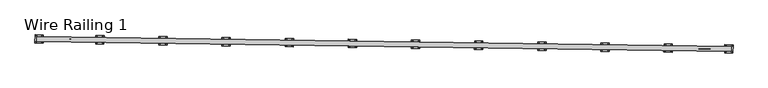
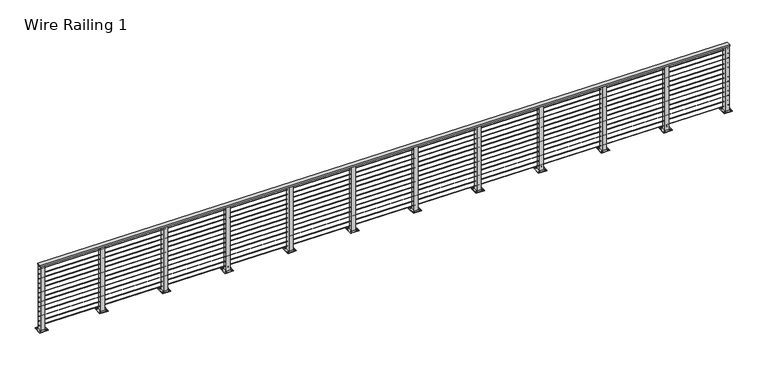
"""IFC4 building model written with IfcOpenShell, lengths in millimetres: railing geometry, Wire Railing 1."""

from ifc_helpers import new_model, si_unit, point, frame, frame_2d, origin, place, context, project, spatial, polyline, circle_curve, trimmed, segment, composite_curve, outline, extrude, source, transform, mapped, element, save


def wire_railing_1_a902e167(model_context):
    return source(origin(), model_context, "Body", "SweptSolid", [
        extrude(outline(polyline([(35445.2454193, 41277.4063498), (35446.3492316, 41353.5983546), (45957.1135693, 41201.326324), (45956.009757, 41125.1343191), (35445.2454193, 41277.4063498)])), frame((0.0, 0.0, 267138.15), z_axis=(0.0, 0.0, 1.0), x_axis=(1.0, 0.0, 0.0)), (0.0, 0.0, 1.0), 19.05),
        extrude(outline(composite_curve([segment(trimmed(circle_curve(frame_2d((0.0, 2.38125)), 2.38125), [point((2.3812499, 2.38125))], [point((-2.3812501, 2.38125))], False, "CARTESIAN"), True, "CONTINUOUS"), segment(trimmed(circle_curve(frame_2d((0.0, 2.38125)), 2.38125), [point((-2.3812501, 2.38125))], [point((2.3812499, 2.38125))], False, "CARTESIAN"), True, "CONTINUOUS")], self_intersect=False)), frame((45956.5616632, 41163.2303216, 267081.0), z_axis=(-0.9998950763646337, 0.014485726138629394, 0.0), x_axis=(0.014485726138629394, 0.9998950763646337, 0.0)), (0.0, 0.0, 1.0), 10511.8672811),
        extrude(outline(composite_curve([segment(trimmed(circle_curve(frame_2d((0.0, 2.38125)), 2.38125), [point((2.3812499, 2.38125))], [point((-2.3812501, 2.38125))], False, "CARTESIAN"), True, "CONTINUOUS"), segment(trimmed(circle_curve(frame_2d((0.0, 2.38125)), 2.38125), [point((-2.3812501, 2.38125))], [point((2.3812499, 2.38125))], False, "CARTESIAN"), True, "CONTINUOUS")], self_intersect=False)), frame((45956.5616632, 41163.2303216, 267004.8), z_axis=(-0.9998950763646337, 0.014485726138629394, 0.0), x_axis=(0.014485726138629394, 0.9998950763646337, 0.0)), (0.0, 0.0, 1.0), 10511.8672811),
        extrude(outline(composite_curve([segment(trimmed(circle_curve(frame_2d((0.0, 2.38125)), 2.38125), [point((2.3812499, 2.38125))], [point((-2.3812501, 2.38125))], False, "CARTESIAN"), True, "CONTINUOUS"), segment(trimmed(circle_curve(frame_2d((0.0, 2.38125)), 2.38125), [point((-2.3812501, 2.38125))], [point((2.3812499, 2.38125))], False, "CARTESIAN"), True, "CONTINUOUS")], self_intersect=False)), frame((45956.5616632, 41163.2303216, 266928.6), z_axis=(-0.9998950763646337, 0.014485726138629394, 0.0), x_axis=(0.014485726138629394, 0.9998950763646337, 0.0)), (0.0, 0.0, 1.0), 10511.8672811),
        extrude(outline(composite_curve([segment(trimmed(circle_curve(frame_2d((0.0, 2.38125)), 2.38125), [point((2.3812499, 2.38125))], [point((-2.3812501, 2.38125))], False, "CARTESIAN"), True, "CONTINUOUS"), segment(trimmed(circle_curve(frame_2d((0.0, 2.38125)), 2.38125), [point((-2.3812501, 2.38125))], [point((2.3812499, 2.38125))], False, "CARTESIAN"), True, "CONTINUOUS")], self_intersect=False)), frame((45956.5616632, 41163.2303216, 266852.4), z_axis=(-0.9998950763646337, 0.014485726138629394, 0.0), x_axis=(0.014485726138629394, 0.9998950763646337, 0.0)), (0.0, 0.0, 1.0), 10511.8672811),
        extrude(outline(composite_curve([segment(trimmed(circle_curve(frame_2d((0.0, 2.38125)), 2.38125), [point((2.3812499, 2.38125))], [point((-2.3812501, 2.38125))], False, "CARTESIAN"), True, "CONTINUOUS"), segment(trimmed(circle_curve(frame_2d((0.0, 2.38125)), 2.38125), [point((-2.3812501, 2.38125))], [point((2.3812499, 2.38125))], False, "CARTESIAN"), True, "CONTINUOUS")], self_intersect=False)), frame((45956.5616632, 41163.2303216, 266776.2), z_axis=(-0.9998950763646337, 0.014485726138629394, 0.0), x_axis=(0.014485726138629394, 0.9998950763646337, 0.0)), (0.0, 0.0, 1.0), 10511.8672811),
        extrude(outline(composite_curve([segment(trimmed(circle_curve(frame_2d((0.0, 2.38125)), 2.38125), [point((2.3812499, 2.38125))], [point((-2.3812501, 2.38125))], False, "CARTESIAN"), True, "CONTINUOUS"), segment(trimmed(circle_curve(frame_2d((0.0, 2.38125)), 2.38125), [point((-2.3812501, 2.38125))], [point((2.3812499, 2.38125))], False, "CARTESIAN"), True, "CONTINUOUS")], self_intersect=False)), frame((45956.5616632, 41163.2303216, 266700.0), z_axis=(-0.9998950763646337, 0.014485726138629394, 0.0), x_axis=(0.014485726138629394, 0.9998950763646337, 0.0)), (0.0, 0.0, 1.0), 10511.8672811),
        extrude(outline(composite_curve([segment(trimmed(circle_curve(frame_2d((0.0, 2.38125)), 2.38125), [point((2.3812499, 2.38125))], [point((-2.3812501, 2.38125))], False, "CARTESIAN"), True, "CONTINUOUS"), segment(trimmed(circle_curve(frame_2d((0.0, 2.38125)), 2.38125), [point((-2.3812501, 2.38125))], [point((2.3812499, 2.38125))], False, "CARTESIAN"), True, "CONTINUOUS")], self_intersect=False)), frame((45956.5616632, 41163.2303216, 266623.8), z_axis=(-0.9998950763646337, 0.014485726138629394, 0.0), x_axis=(0.014485726138629394, 0.9998950763646337, 0.0)), (0.0, 0.0, 1.0), 10511.8672811),
        extrude(outline(composite_curve([segment(trimmed(circle_curve(frame_2d((0.0, 2.38125)), 2.38125), [point((2.3812499, 2.38125))], [point((-2.3812501, 2.38125))], False, "CARTESIAN"), True, "CONTINUOUS"), segment(trimmed(circle_curve(frame_2d((0.0, 2.38125)), 2.38125), [point((-2.3812501, 2.38125))], [point((2.3812499, 2.38125))], False, "CARTESIAN"), True, "CONTINUOUS")], self_intersect=False)), frame((45956.5616632, 41163.2303216, 266547.6), z_axis=(-0.9998950763646337, 0.014485726138629394, 0.0), x_axis=(0.014485726138629394, 0.9998950763646337, 0.0)), (0.0, 0.0, 1.0), 10511.8672811),
        extrude(outline(composite_curve([segment(trimmed(circle_curve(frame_2d((0.0, 2.38125)), 2.38125), [point((2.3812499, 2.38125))], [point((-2.3812501, 2.38125))], False, "CARTESIAN"), True, "CONTINUOUS"), segment(trimmed(circle_curve(frame_2d((0.0, 2.38125)), 2.38125), [point((-2.3812501, 2.38125))], [point((2.3812499, 2.38125))], False, "CARTESIAN"), True, "CONTINUOUS")], self_intersect=False)), frame((45956.5616632, 41163.2303216, 266471.4), z_axis=(-0.9998950763646337, 0.014485726138629394, 0.0), x_axis=(0.014485726138629394, 0.9998950763646337, 0.0)), (0.0, 0.0, 1.0), 10511.8672811),
        extrude(outline(composite_curve([segment(trimmed(circle_curve(frame_2d((0.0, 2.38125)), 2.38125), [point((2.3812499, 2.38125))], [point((-2.3812501, 2.38125))], False, "CARTESIAN"), True, "CONTINUOUS"), segment(trimmed(circle_curve(frame_2d((0.0, 2.38125)), 2.38125), [point((-2.3812501, 2.38125))], [point((2.3812499, 2.38125))], False, "CARTESIAN"), True, "CONTINUOUS")], self_intersect=False)), frame((45956.5616632, 41163.2303216, 266395.2), z_axis=(-0.9998950763646337, 0.014485726138629394, 0.0), x_axis=(0.014485726138629394, 0.9998950763646337, 0.0)), (0.0, 0.0, 1.0), 10511.8672811),
        extrude(outline(composite_curve([segment(trimmed(circle_curve(frame_2d((0.0, 2.38125)), 2.38125), [point((2.3812499, 2.38125))], [point((-2.3812501, 2.38125))], False, "CARTESIAN"), True, "CONTINUOUS"), segment(trimmed(circle_curve(frame_2d((0.0, 2.38125)), 2.38125), [point((-2.3812501, 2.38125))], [point((2.3812499, 2.38125))], False, "CARTESIAN"), True, "CONTINUOUS")], self_intersect=False)), frame((45956.5616632, 41163.2303216, 266319.0), z_axis=(-0.9998950763646337, 0.014485726138629394, 0.0), x_axis=(0.014485726138629394, 0.9998950763646337, 0.0)), (0.0, 0.0, 1.0), 10511.8672811),
        extrude(outline(composite_curve([segment(trimmed(circle_curve(frame_2d((0.0, 2.38125)), 2.38125), [point((2.3812499, 2.38125))], [point((-2.3812501, 2.38125))], False, "CARTESIAN"), True, "CONTINUOUS"), segment(trimmed(circle_curve(frame_2d((0.0, 2.38125)), 2.38125), [point((-2.3812501, 2.38125))], [point((2.3812499, 2.38125))], False, "CARTESIAN"), True, "CONTINUOUS")], self_intersect=False)), frame((45956.5616632, 41163.2303216, 266242.8), z_axis=(-0.9998950763646337, 0.014485726138629394, 0.0), x_axis=(0.014485726138629394, 0.9998950763646337, 0.0)), (0.0, 0.0, 1.0), 10511.8672811),
        extrude(outline(composite_curve([segment(trimmed(circle_curve(frame_2d((0.0, 2.38125)), 2.38125), [point((2.3812499, 2.38125))], [point((-2.3812501, 2.38125))], False, "CARTESIAN"), True, "CONTINUOUS"), segment(trimmed(circle_curve(frame_2d((0.0, 2.38125)), 2.38125), [point((-2.3812501, 2.38125))], [point((2.3812499, 2.38125))], False, "CARTESIAN"), True, "CONTINUOUS")], self_intersect=False)), frame((45956.5616632, 41163.2303216, 266166.6), z_axis=(-0.9998950763646337, 0.014485726138629394, 0.0), x_axis=(0.014485726138629394, 0.9998950763646337, 0.0)), (0.0, 0.0, 1.0), 10511.8672811),
        extrude(outline(composite_curve([segment(trimmed(circle_curve(frame_2d((44955.9484058, 41133.2717878)), 6.35), [point((44955.8564214, 41126.9224541))], [point((44956.0403902, 41139.6211215))], False, "CARTESIAN"), True, "CONTINUOUS"), segment(trimmed(circle_curve(frame_2d((44955.9484058, 41133.2717878)), 6.35), [point((44956.0403902, 41139.6211215))], [point((44955.8564214, 41126.9224541))], False, "CARTESIAN"), True, "CONTINUOUS")], self_intersect=False)), frame((0.0, 0.0, 266090.4), z_axis=(0.0, 0.0, 1.0), x_axis=(1.0, 0.0, 0.0)), (0.0, 0.0, 1.0), 12.7),
        extrude(outline(composite_curve([segment(trimmed(circle_curve(frame_2d((44957.2361869, 41222.1624601)), 6.35), [point((44957.1442025, 41215.8131264))], [point((44957.3281712, 41228.5117938))], False, "CARTESIAN"), True, "CONTINUOUS"), segment(trimmed(circle_curve(frame_2d((44957.2361869, 41222.1624601)), 6.35), [point((44957.3281712, 41228.5117938))], [point((44957.1442025, 41215.8131264))], False, "CARTESIAN"), True, "CONTINUOUS")], self_intersect=False)), frame((0.0, 0.0, 266090.4), z_axis=(0.0, 0.0, 1.0), x_axis=(1.0, 0.0, 0.0)), (0.0, 0.0, 1.0), 12.7),
        extrude(outline(composite_curve([segment(trimmed(circle_curve(frame_2d((45044.8390781, 41131.9840068)), 6.35), [point((45044.7470937, 41125.634673))], [point((45044.9310624, 41138.3333405))], False, "CARTESIAN"), True, "CONTINUOUS"), segment(trimmed(circle_curve(frame_2d((45044.8390781, 41131.9840068)), 6.35), [point((45044.9310624, 41138.3333405))], [point((45044.7470937, 41125.634673))], False, "CARTESIAN"), True, "CONTINUOUS")], self_intersect=False)), frame((0.0, 0.0, 266090.4), z_axis=(0.0, 0.0, 1.0), x_axis=(1.0, 0.0, 0.0)), (0.0, 0.0, 1.0), 12.7),
        extrude(outline(composite_curve([segment(trimmed(circle_curve(frame_2d((45046.1268591, 41220.874679)), 6.35), [point((45046.0348748, 41214.5253453))], [point((45046.2188435, 41227.2240128))], False, "CARTESIAN"), True, "CONTINUOUS"), segment(trimmed(circle_curve(frame_2d((45046.1268591, 41220.874679)), 6.35), [point((45046.2188435, 41227.2240128))], [point((45046.0348748, 41214.5253453))], False, "CARTESIAN"), True, "CONTINUOUS")], self_intersect=False)), frame((0.0, 0.0, 266090.4), z_axis=(0.0, 0.0, 1.0), x_axis=(1.0, 0.0, 0.0)), (0.0, 0.0, 1.0), 12.7),
        extrude(outline(polyline([(44938.4641387, 41241.4864144), (45065.4508134, 41239.6467272), (45063.6111262, 41112.6600525), (44936.6244515, 41114.4997397), (44938.4641387, 41241.4864144)])), frame((0.0, 0.0, 266090.4), z_axis=(0.0, 0.0, 1.0), x_axis=(1.0, 0.0, 0.0)), (0.0, 0.0, 1.0), 6.35),
        extrude(outline(polyline([(44971.3152229, 41207.6694944), (45031.6338934, 41206.795643), (45030.760042, 41146.4769725), (44970.4413715, 41147.3508239), (44971.3152229, 41207.6694944)]), holes=[polyline([(44977.5725723, 41201.2281763), (44976.8826896, 41153.6081733), (45024.5026926, 41152.9182906), (45025.1925753, 41200.5382936), (44977.5725723, 41201.2281763)])]), frame((0.0, 0.0, 266090.4), z_axis=(0.0, 0.0, 1.0), x_axis=(1.0, 0.0, 0.0)), (0.0, 0.0, 1.0), 1047.75),
        extrude(outline(composite_curve([segment(trimmed(circle_curve(frame_2d((44000.4243751, 41147.1146997)), 6.35), [point((44000.3323907, 41140.765366))], [point((44000.5163595, 41153.4640334))], False, "CARTESIAN"), True, "CONTINUOUS"), segment(trimmed(circle_curve(frame_2d((44000.4243751, 41147.1146997)), 6.35), [point((44000.5163595, 41153.4640334))], [point((44000.3323907, 41140.765366))], False, "CARTESIAN"), True, "CONTINUOUS")], self_intersect=False)), frame((0.0, 0.0, 266090.4), z_axis=(0.0, 0.0, 1.0), x_axis=(1.0, 0.0, 0.0)), (0.0, 0.0, 1.0), 12.7),
        extrude(outline(composite_curve([segment(trimmed(circle_curve(frame_2d((44001.7121561, 41236.005372)), 6.35), [point((44001.6201718, 41229.6560382))], [point((44001.8041405, 41242.3547057))], False, "CARTESIAN"), True, "CONTINUOUS"), segment(trimmed(circle_curve(frame_2d((44001.7121561, 41236.005372)), 6.35), [point((44001.8041405, 41242.3547057))], [point((44001.6201718, 41229.6560382))], False, "CARTESIAN"), True, "CONTINUOUS")], self_intersect=False)), frame((0.0, 0.0, 266090.4), z_axis=(0.0, 0.0, 1.0), x_axis=(1.0, 0.0, 0.0)), (0.0, 0.0, 1.0), 12.7),
        extrude(outline(composite_curve([segment(trimmed(circle_curve(frame_2d((44089.3150474, 41145.8269186)), 6.35), [point((44089.223063, 41139.4775849))], [point((44089.4070317, 41152.1762524))], False, "CARTESIAN"), True, "CONTINUOUS"), segment(trimmed(circle_curve(frame_2d((44089.3150474, 41145.8269186)), 6.35), [point((44089.4070317, 41152.1762524))], [point((44089.223063, 41139.4775849))], False, "CARTESIAN"), True, "CONTINUOUS")], self_intersect=False)), frame((0.0, 0.0, 266090.4), z_axis=(0.0, 0.0, 1.0), x_axis=(1.0, 0.0, 0.0)), (0.0, 0.0, 1.0), 12.7),
        extrude(outline(composite_curve([segment(trimmed(circle_curve(frame_2d((44090.6028284, 41234.7175909)), 6.35), [point((44090.5108441, 41228.3682572))], [point((44090.6948128, 41241.0669247))], False, "CARTESIAN"), True, "CONTINUOUS"), segment(trimmed(circle_curve(frame_2d((44090.6028284, 41234.7175909)), 6.35), [point((44090.6948128, 41241.0669247))], [point((44090.5108441, 41228.3682572))], False, "CARTESIAN"), True, "CONTINUOUS")], self_intersect=False)), frame((0.0, 0.0, 266090.4), z_axis=(0.0, 0.0, 1.0), x_axis=(1.0, 0.0, 0.0)), (0.0, 0.0, 1.0), 12.7),
        extrude(outline(polyline([(43982.940108, 41255.3293263), (44109.9267827, 41253.489639), (44108.0870955, 41126.5029643), (43981.1004208, 41128.3426516), (43982.940108, 41255.3293263)])), frame((0.0, 0.0, 266090.4), z_axis=(0.0, 0.0, 1.0), x_axis=(1.0, 0.0, 0.0)), (0.0, 0.0, 1.0), 6.35),
        extrude(outline(polyline([(44015.7911922, 41221.5124063), (44076.1098627, 41220.6385548), (44075.2360113, 41160.3198844), (44014.9173408, 41161.1937358), (44015.7911922, 41221.5124063)]), holes=[polyline([(44022.0485416, 41215.0710882), (44021.3586589, 41167.4510852), (44068.9786619, 41166.7612024), (44069.6685446, 41214.3812055), (44022.0485416, 41215.0710882)])]), frame((0.0, 0.0, 266090.4), z_axis=(0.0, 0.0, 1.0), x_axis=(1.0, 0.0, 0.0)), (0.0, 0.0, 1.0), 1047.75),
        extrude(outline(composite_curve([segment(trimmed(circle_curve(frame_2d((43044.9003444, 41160.9576116)), 6.35), [point((43044.80836, 41154.6082778))], [point((43044.9923287, 41167.3069453))], False, "CARTESIAN"), True, "CONTINUOUS"), segment(trimmed(circle_curve(frame_2d((43044.9003444, 41160.9576116)), 6.35), [point((43044.9923287, 41167.3069453))], [point((43044.80836, 41154.6082778))], False, "CARTESIAN"), True, "CONTINUOUS")], self_intersect=False)), frame((0.0, 0.0, 266090.4), z_axis=(0.0, 0.0, 1.0), x_axis=(1.0, 0.0, 0.0)), (0.0, 0.0, 1.0), 12.7),
        extrude(outline(composite_curve([segment(trimmed(circle_curve(frame_2d((43046.1881254, 41249.8482839)), 6.35), [point((43046.0961411, 41243.4989501))], [point((43046.2801098, 41256.1976176))], False, "CARTESIAN"), True, "CONTINUOUS"), segment(trimmed(circle_curve(frame_2d((43046.1881254, 41249.8482839)), 6.35), [point((43046.2801098, 41256.1976176))], [point((43046.0961411, 41243.4989501))], False, "CARTESIAN"), True, "CONTINUOUS")], self_intersect=False)), frame((0.0, 0.0, 266090.4), z_axis=(0.0, 0.0, 1.0), x_axis=(1.0, 0.0, 0.0)), (0.0, 0.0, 1.0), 12.7),
        extrude(outline(composite_curve([segment(trimmed(circle_curve(frame_2d((43133.7910167, 41159.6698305)), 6.35), [point((43133.6990323, 41153.3204968))], [point((43133.883001, 41166.0191642))], False, "CARTESIAN"), True, "CONTINUOUS"), segment(trimmed(circle_curve(frame_2d((43133.7910167, 41159.6698305)), 6.35), [point((43133.883001, 41166.0191642))], [point((43133.6990323, 41153.3204968))], False, "CARTESIAN"), True, "CONTINUOUS")], self_intersect=False)), frame((0.0, 0.0, 266090.4), z_axis=(0.0, 0.0, 1.0), x_axis=(1.0, 0.0, 0.0)), (0.0, 0.0, 1.0), 12.7),
        extrude(outline(composite_curve([segment(trimmed(circle_curve(frame_2d((43135.0787977, 41248.5605028)), 6.35), [point((43134.9868134, 41242.2111691))], [point((43135.1707821, 41254.9098365))], False, "CARTESIAN"), True, "CONTINUOUS"), segment(trimmed(circle_curve(frame_2d((43135.0787977, 41248.5605028)), 6.35), [point((43135.1707821, 41254.9098365))], [point((43134.9868134, 41242.2111691))], False, "CARTESIAN"), True, "CONTINUOUS")], self_intersect=False)), frame((0.0, 0.0, 266090.4), z_axis=(0.0, 0.0, 1.0), x_axis=(1.0, 0.0, 0.0)), (0.0, 0.0, 1.0), 12.7),
        extrude(outline(polyline([(43027.4160773, 41269.1722381), (43154.402752, 41267.3325509), (43152.5630648, 41140.3458762), (43025.5763901, 41142.1855634), (43027.4160773, 41269.1722381)])), frame((0.0, 0.0, 266090.4), z_axis=(0.0, 0.0, 1.0), x_axis=(1.0, 0.0, 0.0)), (0.0, 0.0, 1.0), 6.35),
        extrude(outline(polyline([(43060.2671615, 41235.3553181), (43120.585832, 41234.4814667), (43119.7119806, 41174.1627962), (43059.3933101, 41175.0366477), (43060.2671615, 41235.3553181)]), holes=[polyline([(43066.5245109, 41228.914), (43065.8346282, 41181.293997), (43113.4546312, 41180.6041143), (43114.1445139, 41228.2241173), (43066.5245109, 41228.914)])]), frame((0.0, 0.0, 266090.4), z_axis=(0.0, 0.0, 1.0), x_axis=(1.0, 0.0, 0.0)), (0.0, 0.0, 1.0), 1047.75),
        extrude(outline(composite_curve([segment(trimmed(circle_curve(frame_2d((42089.3763137, 41174.8005234)), 6.35), [point((42089.2843293, 41168.4511897))], [point((42089.468298, 41181.1498572))], False, "CARTESIAN"), True, "CONTINUOUS"), segment(trimmed(circle_curve(frame_2d((42089.3763137, 41174.8005234)), 6.35), [point((42089.468298, 41181.1498572))], [point((42089.2843293, 41168.4511897))], False, "CARTESIAN"), True, "CONTINUOUS")], self_intersect=False)), frame((0.0, 0.0, 266090.4), z_axis=(0.0, 0.0, 1.0), x_axis=(1.0, 0.0, 0.0)), (0.0, 0.0, 1.0), 12.7),
        extrude(outline(composite_curve([segment(trimmed(circle_curve(frame_2d((42090.6640947, 41263.6911957)), 6.35), [point((42090.5721104, 41257.341862))], [point((42090.7560791, 41270.0405295))], False, "CARTESIAN"), True, "CONTINUOUS"), segment(trimmed(circle_curve(frame_2d((42090.6640947, 41263.6911957)), 6.35), [point((42090.7560791, 41270.0405295))], [point((42090.5721104, 41257.341862))], False, "CARTESIAN"), True, "CONTINUOUS")], self_intersect=False)), frame((0.0, 0.0, 266090.4), z_axis=(0.0, 0.0, 1.0), x_axis=(1.0, 0.0, 0.0)), (0.0, 0.0, 1.0), 12.7),
        extrude(outline(composite_curve([segment(trimmed(circle_curve(frame_2d((42178.266986, 41173.5127424)), 6.35), [point((42178.1750016, 41167.1634087))], [point((42178.3589703, 41179.8620761))], False, "CARTESIAN"), True, "CONTINUOUS"), segment(trimmed(circle_curve(frame_2d((42178.266986, 41173.5127424)), 6.35), [point((42178.3589703, 41179.8620761))], [point((42178.1750016, 41167.1634087))], False, "CARTESIAN"), True, "CONTINUOUS")], self_intersect=False)), frame((0.0, 0.0, 266090.4), z_axis=(0.0, 0.0, 1.0), x_axis=(1.0, 0.0, 0.0)), (0.0, 0.0, 1.0), 12.7),
        extrude(outline(composite_curve([segment(trimmed(circle_curve(frame_2d((42179.554767, 41262.4034147)), 6.35), [point((42179.4627827, 41256.0540809))], [point((42179.6467514, 41268.7527484))], False, "CARTESIAN"), True, "CONTINUOUS"), segment(trimmed(circle_curve(frame_2d((42179.554767, 41262.4034147)), 6.35), [point((42179.6467514, 41268.7527484))], [point((42179.4627827, 41256.0540809))], False, "CARTESIAN"), True, "CONTINUOUS")], self_intersect=False)), frame((0.0, 0.0, 266090.4), z_axis=(0.0, 0.0, 1.0), x_axis=(1.0, 0.0, 0.0)), (0.0, 0.0, 1.0), 12.7),
        extrude(outline(polyline([(42071.8920466, 41283.01515), (42198.8787213, 41281.1754628), (42197.0390341, 41154.1887881), (42070.0523594, 41156.0284753), (42071.8920466, 41283.01515)])), frame((0.0, 0.0, 266090.4), z_axis=(0.0, 0.0, 1.0), x_axis=(1.0, 0.0, 0.0)), (0.0, 0.0, 1.0), 6.35),
        extrude(outline(polyline([(42104.7431308, 41249.19823), (42165.0618013, 41248.3243786), (42164.1879499, 41188.0057081), (42103.8692794, 41188.8795595), (42104.7431308, 41249.19823)]), holes=[polyline([(42111.0004802, 41242.7569119), (42110.3105975, 41195.1369089), (42157.9306005, 41194.4470262), (42158.6204832, 41242.0670292), (42111.0004802, 41242.7569119)])]), frame((0.0, 0.0, 266090.4), z_axis=(0.0, 0.0, 1.0), x_axis=(1.0, 0.0, 0.0)), (0.0, 0.0, 1.0), 1047.75),
        extrude(outline(composite_curve([segment(trimmed(circle_curve(frame_2d((41133.852283, 41188.6434353)), 6.35), [point((41133.7602986, 41182.2941016))], [point((41133.9442673, 41194.9927691))], False, "CARTESIAN"), True, "CONTINUOUS"), segment(trimmed(circle_curve(frame_2d((41133.852283, 41188.6434353)), 6.35), [point((41133.9442673, 41194.9927691))], [point((41133.7602986, 41182.2941016))], False, "CARTESIAN"), True, "CONTINUOUS")], self_intersect=False)), frame((0.0, 0.0, 266090.4), z_axis=(0.0, 0.0, 1.0), x_axis=(1.0, 0.0, 0.0)), (0.0, 0.0, 1.0), 12.7),
        extrude(outline(composite_curve([segment(trimmed(circle_curve(frame_2d((41135.140064, 41277.5341076)), 6.35), [point((41135.0480797, 41271.1847739))], [point((41135.2320484, 41283.8834413))], False, "CARTESIAN"), True, "CONTINUOUS"), segment(trimmed(circle_curve(frame_2d((41135.140064, 41277.5341076)), 6.35), [point((41135.2320484, 41283.8834413))], [point((41135.0480797, 41271.1847739))], False, "CARTESIAN"), True, "CONTINUOUS")], self_intersect=False)), frame((0.0, 0.0, 266090.4), z_axis=(0.0, 0.0, 1.0), x_axis=(1.0, 0.0, 0.0)), (0.0, 0.0, 1.0), 12.7),
        extrude(outline(composite_curve([segment(trimmed(circle_curve(frame_2d((41222.7429553, 41187.3556543)), 6.35), [point((41222.6509709, 41181.0063205))], [point((41222.8349396, 41193.704988))], False, "CARTESIAN"), True, "CONTINUOUS"), segment(trimmed(circle_curve(frame_2d((41222.7429553, 41187.3556543)), 6.35), [point((41222.8349396, 41193.704988))], [point((41222.6509709, 41181.0063205))], False, "CARTESIAN"), True, "CONTINUOUS")], self_intersect=False)), frame((0.0, 0.0, 266090.4), z_axis=(0.0, 0.0, 1.0), x_axis=(1.0, 0.0, 0.0)), (0.0, 0.0, 1.0), 12.7),
        extrude(outline(composite_curve([segment(trimmed(circle_curve(frame_2d((41224.0307363, 41276.2463266)), 6.35), [point((41223.938752, 41269.8969928))], [point((41224.1227207, 41282.5956603))], False, "CARTESIAN"), True, "CONTINUOUS"), segment(trimmed(circle_curve(frame_2d((41224.0307363, 41276.2463266)), 6.35), [point((41224.1227207, 41282.5956603))], [point((41223.938752, 41269.8969928))], False, "CARTESIAN"), True, "CONTINUOUS")], self_intersect=False)), frame((0.0, 0.0, 266090.4), z_axis=(0.0, 0.0, 1.0), x_axis=(1.0, 0.0, 0.0)), (0.0, 0.0, 1.0), 12.7),
        extrude(outline(polyline([(41116.3680159, 41296.8580619), (41243.3546906, 41295.0183747), (41241.5150034, 41168.0317), (41114.5283287, 41169.8713872), (41116.3680159, 41296.8580619)])), frame((0.0, 0.0, 266090.4), z_axis=(0.0, 0.0, 1.0), x_axis=(1.0, 0.0, 0.0)), (0.0, 0.0, 1.0), 6.35),
        extrude(outline(polyline([(41149.2191001, 41263.0411419), (41209.5377706, 41262.1672905), (41208.6639192, 41201.84862), (41148.3452487, 41202.7224714), (41149.2191001, 41263.0411419)]), holes=[polyline([(41155.4764495, 41256.5998238), (41154.7865668, 41208.9798208), (41202.4065698, 41208.2899381), (41203.0964525, 41255.9099411), (41155.4764495, 41256.5998238)])]), frame((0.0, 0.0, 266090.4), z_axis=(0.0, 0.0, 1.0), x_axis=(1.0, 0.0, 0.0)), (0.0, 0.0, 1.0), 1047.75),
        extrude(outline(composite_curve([segment(trimmed(circle_curve(frame_2d((40178.3282523, 41202.4863472)), 6.35), [point((40178.2362679, 41196.1370135))], [point((40178.4202366, 41208.8356809))], False, "CARTESIAN"), True, "CONTINUOUS"), segment(trimmed(circle_curve(frame_2d((40178.3282523, 41202.4863472)), 6.35), [point((40178.4202366, 41208.8356809))], [point((40178.2362679, 41196.1370135))], False, "CARTESIAN"), True, "CONTINUOUS")], self_intersect=False)), frame((0.0, 0.0, 266090.4), z_axis=(0.0, 0.0, 1.0), x_axis=(1.0, 0.0, 0.0)), (0.0, 0.0, 1.0), 12.7),
        extrude(outline(composite_curve([segment(trimmed(circle_curve(frame_2d((40179.6160333, 41291.3770195)), 6.35), [point((40179.524049, 41285.0276857))], [point((40179.7080177, 41297.7263532))], False, "CARTESIAN"), True, "CONTINUOUS"), segment(trimmed(circle_curve(frame_2d((40179.6160333, 41291.3770195)), 6.35), [point((40179.7080177, 41297.7263532))], [point((40179.524049, 41285.0276857))], False, "CARTESIAN"), True, "CONTINUOUS")], self_intersect=False)), frame((0.0, 0.0, 266090.4), z_axis=(0.0, 0.0, 1.0), x_axis=(1.0, 0.0, 0.0)), (0.0, 0.0, 1.0), 12.7),
        extrude(outline(composite_curve([segment(trimmed(circle_curve(frame_2d((40267.2189246, 41201.1985661)), 6.35), [point((40267.1269402, 41194.8492324))], [point((40267.3109089, 41207.5478999))], False, "CARTESIAN"), True, "CONTINUOUS"), segment(trimmed(circle_curve(frame_2d((40267.2189246, 41201.1985661)), 6.35), [point((40267.3109089, 41207.5478999))], [point((40267.1269402, 41194.8492324))], False, "CARTESIAN"), True, "CONTINUOUS")], self_intersect=False)), frame((0.0, 0.0, 266090.4), z_axis=(0.0, 0.0, 1.0), x_axis=(1.0, 0.0, 0.0)), (0.0, 0.0, 1.0), 12.7),
        extrude(outline(composite_curve([segment(trimmed(circle_curve(frame_2d((40268.5067056, 41290.0892384)), 6.35), [point((40268.4147213, 41283.7399047))], [point((40268.59869, 41296.4385722))], False, "CARTESIAN"), True, "CONTINUOUS"), segment(trimmed(circle_curve(frame_2d((40268.5067056, 41290.0892384)), 6.35), [point((40268.59869, 41296.4385722))], [point((40268.4147213, 41283.7399047))], False, "CARTESIAN"), True, "CONTINUOUS")], self_intersect=False)), frame((0.0, 0.0, 266090.4), z_axis=(0.0, 0.0, 1.0), x_axis=(1.0, 0.0, 0.0)), (0.0, 0.0, 1.0), 12.7),
        extrude(outline(polyline([(40160.8439852, 41310.7009738), (40287.8306599, 41308.8612866), (40285.9909727, 41181.8746119), (40159.004298, 41183.7142991), (40160.8439852, 41310.7009738)])), frame((0.0, 0.0, 266090.4), z_axis=(0.0, 0.0, 1.0), x_axis=(1.0, 0.0, 0.0)), (0.0, 0.0, 1.0), 6.35),
        extrude(outline(polyline([(40193.6950694, 41276.8840538), (40254.0137399, 41276.0102023), (40253.1398885, 41215.6915319), (40192.821218, 41216.5653833), (40193.6950694, 41276.8840538)]), holes=[polyline([(40199.9524188, 41270.4427357), (40199.2625361, 41222.8227327), (40246.8825391, 41222.13285), (40247.5724218, 41269.752853), (40199.9524188, 41270.4427357)])]), frame((0.0, 0.0, 266090.4), z_axis=(0.0, 0.0, 1.0), x_axis=(1.0, 0.0, 0.0)), (0.0, 0.0, 1.0), 1047.75),
        extrude(outline(composite_curve([segment(trimmed(circle_curve(frame_2d((39222.8042216, 41216.3292591)), 6.35), [point((39222.7122372, 41209.9799253))], [point((39222.8962059, 41222.6785928))], False, "CARTESIAN"), True, "CONTINUOUS"), segment(trimmed(circle_curve(frame_2d((39222.8042216, 41216.3292591)), 6.35), [point((39222.8962059, 41222.6785928))], [point((39222.7122372, 41209.9799253))], False, "CARTESIAN"), True, "CONTINUOUS")], self_intersect=False)), frame((0.0, 0.0, 266090.4), z_axis=(0.0, 0.0, 1.0), x_axis=(1.0, 0.0, 0.0)), (0.0, 0.0, 1.0), 12.7),
        extrude(outline(composite_curve([segment(trimmed(circle_curve(frame_2d((39224.0920026, 41305.2199314)), 6.35), [point((39224.0000183, 41298.8705976))], [point((39224.183987, 41311.5692651))], False, "CARTESIAN"), True, "CONTINUOUS"), segment(trimmed(circle_curve(frame_2d((39224.0920026, 41305.2199314)), 6.35), [point((39224.183987, 41311.5692651))], [point((39224.0000183, 41298.8705976))], False, "CARTESIAN"), True, "CONTINUOUS")], self_intersect=False)), frame((0.0, 0.0, 266090.4), z_axis=(0.0, 0.0, 1.0), x_axis=(1.0, 0.0, 0.0)), (0.0, 0.0, 1.0), 12.7),
        extrude(outline(composite_curve([segment(trimmed(circle_curve(frame_2d((39311.6948939, 41215.041478)), 6.35), [point((39311.6029095, 41208.6921443))], [point((39311.7868782, 41221.3908118))], False, "CARTESIAN"), True, "CONTINUOUS"), segment(trimmed(circle_curve(frame_2d((39311.6948939, 41215.041478)), 6.35), [point((39311.7868782, 41221.3908118))], [point((39311.6029095, 41208.6921443))], False, "CARTESIAN"), True, "CONTINUOUS")], self_intersect=False)), frame((0.0, 0.0, 266090.4), z_axis=(0.0, 0.0, 1.0), x_axis=(1.0, 0.0, 0.0)), (0.0, 0.0, 1.0), 12.7),
        extrude(outline(composite_curve([segment(trimmed(circle_curve(frame_2d((39312.9826749, 41303.9321503)), 6.35), [point((39312.8906905, 41297.5828166))], [point((39313.0746593, 41310.281484))], False, "CARTESIAN"), True, "CONTINUOUS"), segment(trimmed(circle_curve(frame_2d((39312.9826749, 41303.9321503)), 6.35), [point((39313.0746593, 41310.281484))], [point((39312.8906905, 41297.5828166))], False, "CARTESIAN"), True, "CONTINUOUS")], self_intersect=False)), frame((0.0, 0.0, 266090.4), z_axis=(0.0, 0.0, 1.0), x_axis=(1.0, 0.0, 0.0)), (0.0, 0.0, 1.0), 12.7),
        extrude(outline(polyline([(39205.3199545, 41324.5438856), (39332.3066292, 41322.7041984), (39330.466942, 41195.7175237), (39203.4802673, 41197.5572109), (39205.3199545, 41324.5438856)])), frame((0.0, 0.0, 266090.4), z_axis=(0.0, 0.0, 1.0), x_axis=(1.0, 0.0, 0.0)), (0.0, 0.0, 1.0), 6.35),
        extrude(outline(polyline([(39238.1710387, 41290.7269656), (39298.4897092, 41289.8531142), (39297.6158578, 41229.5344437), (39237.2971873, 41230.4082952), (39238.1710387, 41290.7269656)]), holes=[polyline([(39244.4283881, 41284.2856475), (39243.7385054, 41236.6656445), (39291.3585084, 41235.9757618), (39292.0483911, 41283.5957648), (39244.4283881, 41284.2856475)])]), frame((0.0, 0.0, 266090.4), z_axis=(0.0, 0.0, 1.0), x_axis=(1.0, 0.0, 0.0)), (0.0, 0.0, 1.0), 1047.75),
        extrude(outline(composite_curve([segment(trimmed(circle_curve(frame_2d((38267.2801909, 41230.1721709)), 6.35), [point((38267.1882065, 41223.8228372))], [point((38267.3721752, 41236.5215047))], False, "CARTESIAN"), True, "CONTINUOUS"), segment(trimmed(circle_curve(frame_2d((38267.2801909, 41230.1721709)), 6.35), [point((38267.3721752, 41236.5215047))], [point((38267.1882065, 41223.8228372))], False, "CARTESIAN"), True, "CONTINUOUS")], self_intersect=False)), frame((0.0, 0.0, 266090.4), z_axis=(0.0, 0.0, 1.0), x_axis=(1.0, 0.0, 0.0)), (0.0, 0.0, 1.0), 12.7),
        extrude(outline(composite_curve([segment(trimmed(circle_curve(frame_2d((38268.5679719, 41319.0628432)), 6.35), [point((38268.4759876, 41312.7135095))], [point((38268.6599563, 41325.412177))], False, "CARTESIAN"), True, "CONTINUOUS"), segment(trimmed(circle_curve(frame_2d((38268.5679719, 41319.0628432)), 6.35), [point((38268.6599563, 41325.412177))], [point((38268.4759876, 41312.7135095))], False, "CARTESIAN"), True, "CONTINUOUS")], self_intersect=False)), frame((0.0, 0.0, 266090.4), z_axis=(0.0, 0.0, 1.0), x_axis=(1.0, 0.0, 0.0)), (0.0, 0.0, 1.0), 12.7),
        extrude(outline(composite_curve([segment(trimmed(circle_curve(frame_2d((38356.1708632, 41228.8843899)), 6.35), [point((38356.0788788, 41222.5350562))], [point((38356.2628475, 41235.2337236))], False, "CARTESIAN"), True, "CONTINUOUS"), segment(trimmed(circle_curve(frame_2d((38356.1708632, 41228.8843899)), 6.35), [point((38356.2628475, 41235.2337236))], [point((38356.0788788, 41222.5350562))], False, "CARTESIAN"), True, "CONTINUOUS")], self_intersect=False)), frame((0.0, 0.0, 266090.4), z_axis=(0.0, 0.0, 1.0), x_axis=(1.0, 0.0, 0.0)), (0.0, 0.0, 1.0), 12.7),
        extrude(outline(composite_curve([segment(trimmed(circle_curve(frame_2d((38357.4586442, 41317.7750622)), 6.35), [point((38357.3666598, 41311.4257284))], [point((38357.5506286, 41324.1243959))], False, "CARTESIAN"), True, "CONTINUOUS"), segment(trimmed(circle_curve(frame_2d((38357.4586442, 41317.7750622)), 6.35), [point((38357.5506286, 41324.1243959))], [point((38357.3666598, 41311.4257284))], False, "CARTESIAN"), True, "CONTINUOUS")], self_intersect=False)), frame((0.0, 0.0, 266090.4), z_axis=(0.0, 0.0, 1.0), x_axis=(1.0, 0.0, 0.0)), (0.0, 0.0, 1.0), 12.7),
        extrude(outline(polyline([(38249.7959238, 41338.3867975), (38376.7825985, 41336.5471103), (38374.9429113, 41209.5604356), (38247.9562366, 41211.4001228), (38249.7959238, 41338.3867975)])), frame((0.0, 0.0, 266090.4), z_axis=(0.0, 0.0, 1.0), x_axis=(1.0, 0.0, 0.0)), (0.0, 0.0, 1.0), 6.35),
        extrude(outline(polyline([(38282.647008, 41304.5698775), (38342.9656785, 41303.6960261), (38342.0918271, 41243.3773556), (38281.7731566, 41244.251207), (38282.647008, 41304.5698775)]), holes=[polyline([(38288.9043574, 41298.1285594), (38288.2144747, 41250.5085564), (38335.8344777, 41249.8186737), (38336.5243604, 41297.4386767), (38288.9043574, 41298.1285594)])]), frame((0.0, 0.0, 266090.4), z_axis=(0.0, 0.0, 1.0), x_axis=(1.0, 0.0, 0.0)), (0.0, 0.0, 1.0), 1047.75),
        extrude(outline(composite_curve([segment(trimmed(circle_curve(frame_2d((37311.7561602, 41244.0150828)), 6.35), [point((37311.6641758, 41237.6657491))], [point((37311.8481445, 41250.3644166))], False, "CARTESIAN"), True, "CONTINUOUS"), segment(trimmed(circle_curve(frame_2d((37311.7561602, 41244.0150828)), 6.35), [point((37311.8481445, 41250.3644166))], [point((37311.6641758, 41237.6657491))], False, "CARTESIAN"), True, "CONTINUOUS")], self_intersect=False)), frame((0.0, 0.0, 266090.4), z_axis=(0.0, 0.0, 1.0), x_axis=(1.0, 0.0, 0.0)), (0.0, 0.0, 1.0), 12.7),
        extrude(outline(composite_curve([segment(trimmed(circle_curve(frame_2d((37313.0439412, 41332.9057551)), 6.35), [point((37312.9519569, 41326.5564214))], [point((37313.1359256, 41339.2550888))], False, "CARTESIAN"), True, "CONTINUOUS"), segment(trimmed(circle_curve(frame_2d((37313.0439412, 41332.9057551)), 6.35), [point((37313.1359256, 41339.2550888))], [point((37312.9519569, 41326.5564214))], False, "CARTESIAN"), True, "CONTINUOUS")], self_intersect=False)), frame((0.0, 0.0, 266090.4), z_axis=(0.0, 0.0, 1.0), x_axis=(1.0, 0.0, 0.0)), (0.0, 0.0, 1.0), 12.7),
        extrude(outline(composite_curve([segment(trimmed(circle_curve(frame_2d((37400.6468324, 41242.7273018)), 6.35), [point((37400.5548481, 41236.377968))], [point((37400.7388168, 41249.0766355))], False, "CARTESIAN"), True, "CONTINUOUS"), segment(trimmed(circle_curve(frame_2d((37400.6468324, 41242.7273018)), 6.35), [point((37400.7388168, 41249.0766355))], [point((37400.5548481, 41236.377968))], False, "CARTESIAN"), True, "CONTINUOUS")], self_intersect=False)), frame((0.0, 0.0, 266090.4), z_axis=(0.0, 0.0, 1.0), x_axis=(1.0, 0.0, 0.0)), (0.0, 0.0, 1.0), 12.7),
        extrude(outline(composite_curve([segment(trimmed(circle_curve(frame_2d((37401.9346135, 41331.6179741)), 6.35), [point((37401.8426291, 41325.2686403))], [point((37402.0265979, 41337.9673078))], False, "CARTESIAN"), True, "CONTINUOUS"), segment(trimmed(circle_curve(frame_2d((37401.9346135, 41331.6179741)), 6.35), [point((37402.0265979, 41337.9673078))], [point((37401.8426291, 41325.2686403))], False, "CARTESIAN"), True, "CONTINUOUS")], self_intersect=False)), frame((0.0, 0.0, 266090.4), z_axis=(0.0, 0.0, 1.0), x_axis=(1.0, 0.0, 0.0)), (0.0, 0.0, 1.0), 12.7),
        extrude(outline(polyline([(37294.2718931, 41352.2297094), (37421.2585678, 41350.3900222), (37419.4188806, 41223.4033475), (37292.4322059, 41225.2430347), (37294.2718931, 41352.2297094)])), frame((0.0, 0.0, 266090.4), z_axis=(0.0, 0.0, 1.0), x_axis=(1.0, 0.0, 0.0)), (0.0, 0.0, 1.0), 6.35),
        extrude(outline(polyline([(37327.1229773, 41318.4127894), (37387.4416478, 41317.538938), (37386.5677964, 41257.2202675), (37326.2491259, 41258.0941189), (37327.1229773, 41318.4127894)]), holes=[polyline([(37333.3803267, 41311.9714713), (37332.690444, 41264.3514683), (37380.310447, 41263.6615856), (37381.0003297, 41311.2815886), (37333.3803267, 41311.9714713)])]), frame((0.0, 0.0, 266090.4), z_axis=(0.0, 0.0, 1.0), x_axis=(1.0, 0.0, 0.0)), (0.0, 0.0, 1.0), 1047.75),
        extrude(outline(composite_curve([segment(trimmed(circle_curve(frame_2d((36356.2321295, 41257.8579947)), 6.35), [point((36356.1401451, 41251.508661))], [point((36356.3241138, 41264.2073284))], False, "CARTESIAN"), True, "CONTINUOUS"), segment(trimmed(circle_curve(frame_2d((36356.2321295, 41257.8579947)), 6.35), [point((36356.3241138, 41264.2073284))], [point((36356.1401451, 41251.508661))], False, "CARTESIAN"), True, "CONTINUOUS")], self_intersect=False)), frame((0.0, 0.0, 266090.4), z_axis=(0.0, 0.0, 1.0), x_axis=(1.0, 0.0, 0.0)), (0.0, 0.0, 1.0), 12.7),
        extrude(outline(composite_curve([segment(trimmed(circle_curve(frame_2d((36357.5199105, 41346.748667)), 6.35), [point((36357.4279261, 41340.3993333))], [point((36357.6118949, 41353.0980007))], False, "CARTESIAN"), True, "CONTINUOUS"), segment(trimmed(circle_curve(frame_2d((36357.5199105, 41346.748667)), 6.35), [point((36357.6118949, 41353.0980007))], [point((36357.4279261, 41340.3993333))], False, "CARTESIAN"), True, "CONTINUOUS")], self_intersect=False)), frame((0.0, 0.0, 266090.4), z_axis=(0.0, 0.0, 1.0), x_axis=(1.0, 0.0, 0.0)), (0.0, 0.0, 1.0), 12.7),
        extrude(outline(composite_curve([segment(trimmed(circle_curve(frame_2d((36445.1228017, 41256.5702136)), 6.35), [point((36445.0308174, 41250.2208799))], [point((36445.2147861, 41262.9195474))], False, "CARTESIAN"), True, "CONTINUOUS"), segment(trimmed(circle_curve(frame_2d((36445.1228017, 41256.5702136)), 6.35), [point((36445.2147861, 41262.9195474))], [point((36445.0308174, 41250.2208799))], False, "CARTESIAN"), True, "CONTINUOUS")], self_intersect=False)), frame((0.0, 0.0, 266090.4), z_axis=(0.0, 0.0, 1.0), x_axis=(1.0, 0.0, 0.0)), (0.0, 0.0, 1.0), 12.7),
        extrude(outline(composite_curve([segment(trimmed(circle_curve(frame_2d((36446.4105828, 41345.4608859)), 6.35), [point((36446.3185984, 41339.1115522))], [point((36446.5025672, 41351.8102197))], False, "CARTESIAN"), True, "CONTINUOUS"), segment(trimmed(circle_curve(frame_2d((36446.4105828, 41345.4608859)), 6.35), [point((36446.5025672, 41351.8102197))], [point((36446.3185984, 41339.1115522))], False, "CARTESIAN"), True, "CONTINUOUS")], self_intersect=False)), frame((0.0, 0.0, 266090.4), z_axis=(0.0, 0.0, 1.0), x_axis=(1.0, 0.0, 0.0)), (0.0, 0.0, 1.0), 12.7),
        extrude(outline(polyline([(36338.7478624, 41366.0726213), (36465.7345371, 41364.2329341), (36463.8948499, 41237.2462594), (36336.9081752, 41239.0859466), (36338.7478624, 41366.0726213)])), frame((0.0, 0.0, 266090.4), z_axis=(0.0, 0.0, 1.0), x_axis=(1.0, 0.0, 0.0)), (0.0, 0.0, 1.0), 6.35),
        extrude(outline(polyline([(36371.5989466, 41332.2557013), (36431.9176171, 41331.3818498), (36431.0437656, 41271.0631794), (36370.7250952, 41271.9370308), (36371.5989466, 41332.2557013)]), holes=[polyline([(36377.856296, 41325.8143832), (36377.1664133, 41278.1943802), (36424.7864163, 41277.5044975), (36425.476299, 41325.1245005), (36377.856296, 41325.8143832)])]), frame((0.0, 0.0, 266090.4), z_axis=(0.0, 0.0, 1.0), x_axis=(1.0, 0.0, 0.0)), (0.0, 0.0, 1.0), 1047.75),
        extrude(outline(composite_curve([segment(trimmed(circle_curve(frame_2d((45873.3764341, 41119.9807821)), 6.35), [point((45873.2844497, 41113.6314484))], [point((45873.4684185, 41126.3301158))], False, "CARTESIAN"), True, "CONTINUOUS"), segment(trimmed(circle_curve(frame_2d((45873.3764341, 41119.9807821)), 6.35), [point((45873.4684185, 41126.3301158))], [point((45873.2844497, 41113.6314484))], False, "CARTESIAN"), True, "CONTINUOUS")], self_intersect=False)), frame((0.0, 0.0, 266090.4), z_axis=(0.0, 0.0, 1.0), x_axis=(1.0, 0.0, 0.0)), (0.0, 0.0, 1.0), 12.7),
        extrude(outline(composite_curve([segment(trimmed(circle_curve(frame_2d((45874.6642151, 41208.8714544)), 6.35), [point((45874.5722308, 41202.5221207))], [point((45874.7561995, 41215.2207881))], False, "CARTESIAN"), True, "CONTINUOUS"), segment(trimmed(circle_curve(frame_2d((45874.6642151, 41208.8714544)), 6.35), [point((45874.7561995, 41215.2207881))], [point((45874.5722308, 41202.5221207))], False, "CARTESIAN"), True, "CONTINUOUS")], self_intersect=False)), frame((0.0, 0.0, 266090.4), z_axis=(0.0, 0.0, 1.0), x_axis=(1.0, 0.0, 0.0)), (0.0, 0.0, 1.0), 12.7),
        extrude(outline(composite_curve([segment(trimmed(circle_curve(frame_2d((45962.2671064, 41118.693001)), 6.35), [point((45962.175122, 41112.3436673))], [point((45962.3590907, 41125.0423348))], False, "CARTESIAN"), True, "CONTINUOUS"), segment(trimmed(circle_curve(frame_2d((45962.2671064, 41118.693001)), 6.35), [point((45962.3590907, 41125.0423348))], [point((45962.175122, 41112.3436673))], False, "CARTESIAN"), True, "CONTINUOUS")], self_intersect=False)), frame((0.0, 0.0, 266090.4), z_axis=(0.0, 0.0, 1.0), x_axis=(1.0, 0.0, 0.0)), (0.0, 0.0, 1.0), 12.7),
        extrude(outline(composite_curve([segment(trimmed(circle_curve(frame_2d((45963.5548874, 41207.5836733)), 6.35), [point((45963.4629031, 41201.2343396))], [point((45963.6468718, 41213.9330071))], False, "CARTESIAN"), True, "CONTINUOUS"), segment(trimmed(circle_curve(frame_2d((45963.5548874, 41207.5836733)), 6.35), [point((45963.6468718, 41213.9330071))], [point((45963.4629031, 41201.2343396))], False, "CARTESIAN"), True, "CONTINUOUS")], self_intersect=False)), frame((0.0, 0.0, 266090.4), z_axis=(0.0, 0.0, 1.0), x_axis=(1.0, 0.0, 0.0)), (0.0, 0.0, 1.0), 12.7),
        extrude(outline(polyline([(45855.892167, 41228.1954087), (45982.8788417, 41226.3557215), (45981.0391545, 41099.3690468), (45854.0524798, 41101.208734), (45855.892167, 41228.1954087)])), frame((0.0, 0.0, 266090.4), z_axis=(0.0, 0.0, 1.0), x_axis=(1.0, 0.0, 0.0)), (0.0, 0.0, 1.0), 6.35),
        extrude(outline(polyline([(45888.7432512, 41194.3784887), (45949.0619217, 41193.5046372), (45948.1880703, 41133.1859668), (45887.8693998, 41134.0598182), (45888.7432512, 41194.3784887)]), holes=[polyline([(45895.0006006, 41187.9371706), (45894.3107179, 41140.3171676), (45941.9307209, 41139.6272849), (45942.6206036, 41187.2472879), (45895.0006006, 41187.9371706)])]), frame((0.0, 0.0, 266090.4), z_axis=(0.0, 0.0, 1.0), x_axis=(1.0, 0.0, 0.0)), (0.0, 0.0, 1.0), 1047.75),
        extrude(outline(composite_curve([segment(trimmed(circle_curve(frame_2d((35438.8041012, 41271.1490004)), 6.35), [point((35438.7121168, 41264.7996667))], [point((35438.8960855, 41277.4983341))], False, "CARTESIAN"), True, "CONTINUOUS"), segment(trimmed(circle_curve(frame_2d((35438.8041012, 41271.1490004)), 6.35), [point((35438.8960855, 41277.4983341))], [point((35438.7121168, 41264.7996667))], False, "CARTESIAN"), True, "CONTINUOUS")], self_intersect=False)), frame((0.0, 0.0, 266090.4), z_axis=(0.0, 0.0, 1.0), x_axis=(1.0, 0.0, 0.0)), (0.0, 0.0, 1.0), 12.7),
        extrude(outline(composite_curve([segment(trimmed(circle_curve(frame_2d((35440.0918822, 41360.0396727)), 6.35), [point((35439.9998978, 41353.690339))], [point((35440.1838666, 41366.3890064))], False, "CARTESIAN"), True, "CONTINUOUS"), segment(trimmed(circle_curve(frame_2d((35440.0918822, 41360.0396727)), 6.35), [point((35440.1838666, 41366.3890064))], [point((35439.9998978, 41353.690339))], False, "CARTESIAN"), True, "CONTINUOUS")], self_intersect=False)), frame((0.0, 0.0, 266090.4), z_axis=(0.0, 0.0, 1.0), x_axis=(1.0, 0.0, 0.0)), (0.0, 0.0, 1.0), 12.7),
        extrude(outline(composite_curve([segment(trimmed(circle_curve(frame_2d((35527.6947734, 41269.8612194)), 6.35), [point((35527.6027891, 41263.5118856))], [point((35527.7867578, 41276.2105531))], False, "CARTESIAN"), True, "CONTINUOUS"), segment(trimmed(circle_curve(frame_2d((35527.6947734, 41269.8612194)), 6.35), [point((35527.7867578, 41276.2105531))], [point((35527.6027891, 41263.5118856))], False, "CARTESIAN"), True, "CONTINUOUS")], self_intersect=False)), frame((0.0, 0.0, 266090.4), z_axis=(0.0, 0.0, 1.0), x_axis=(1.0, 0.0, 0.0)), (0.0, 0.0, 1.0), 12.7),
        extrude(outline(composite_curve([segment(trimmed(circle_curve(frame_2d((35528.9825545, 41358.7518916)), 6.35), [point((35528.8905701, 41352.4025579))], [point((35529.0745389, 41365.1012254))], False, "CARTESIAN"), True, "CONTINUOUS"), segment(trimmed(circle_curve(frame_2d((35528.9825545, 41358.7518916)), 6.35), [point((35529.0745389, 41365.1012254))], [point((35528.8905701, 41352.4025579))], False, "CARTESIAN"), True, "CONTINUOUS")], self_intersect=False)), frame((0.0, 0.0, 266090.4), z_axis=(0.0, 0.0, 1.0), x_axis=(1.0, 0.0, 0.0)), (0.0, 0.0, 1.0), 12.7),
        extrude(outline(polyline([(35421.3198341, 41379.363627), (35548.3065088, 41377.5239398), (35546.4668216, 41250.5372651), (35419.4801469, 41252.3769523), (35421.3198341, 41379.363627)])), frame((0.0, 0.0, 266090.4), z_axis=(0.0, 0.0, 1.0), x_axis=(1.0, 0.0, 0.0)), (0.0, 0.0, 1.0), 6.35),
        extrude(outline(polyline([(35454.1709183, 41345.546707), (35514.4895888, 41344.6728556), (35513.6157374, 41284.3541851), (35453.2970669, 41285.2280365), (35454.1709183, 41345.546707)]), holes=[polyline([(35460.4282677, 41339.1053889), (35459.738385, 41291.4853859), (35507.358388, 41290.7955032), (35508.0482707, 41338.4155062), (35460.4282677, 41339.1053889)])]), frame((0.0, 0.0, 266090.4), z_axis=(0.0, 0.0, 1.0), x_axis=(1.0, 0.0, 0.0)), (0.0, 0.0, 1.0), 1047.75),
    ])


if __name__ == "__main__":
    model = new_model("IFC4")
    model_context = context("Model", 3, world=origin())
    ifc_project = project(units=[si_unit("LENGTHUNIT", "METRE", prefix="MILLI")], contexts=[model_context])
    site = spatial("IfcSite", under=ifc_project)
    building = spatial("IfcBuilding", under=site)
    placement = place(None, origin())
    wire_railing_1_shape = wire_railing_1_a902e167(model_context)
    element("IfcRailing", 1, ObjectType="Wire Railing 1", at=placement, inside=building, context=model_context, shape_type="MappedRepresentation", body=[
        mapped(wire_railing_1_shape, transform((0.0, 0.0, 0.0), x_axis=(1.0, 0.0, 0.0), y_axis=(0.0, 1.0, 0.0), z_axis=(0.0, 0.0, 1.0))),
    ])
    save(model, "model.ifc")

# Revit data of these elements
# Element 1 (IfcRailing, "Wire Railing 1")
#   Materials on its faces: "WIRE RAILING"
# Materials
#   "WIRE RAILING": class "Metal", colour RGB 244 244 244, transparency 0, Manufacturer = "Kawneer", URL = "http://www.kawneer.com/kawneer/north_america/en/home.asp", Cost = 0
